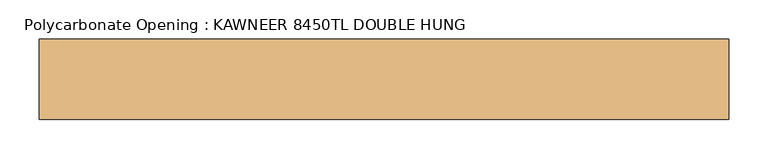
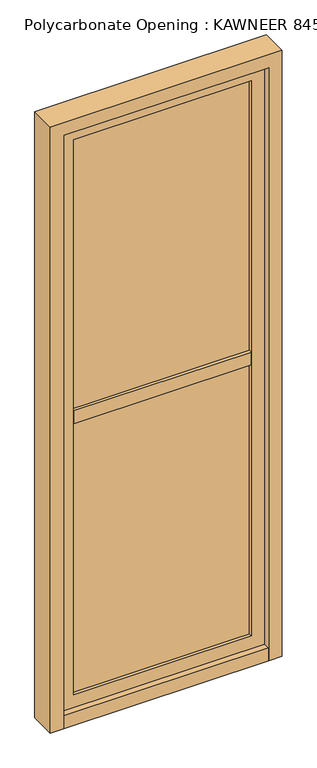
"""IFC4 building model written with IfcOpenShell, lengths in millimetres: door geometry, Polycarbonate Opening : KAWNEER 8450TL DOUBLE HUNG."""

from ifc_helpers import new_model, si_unit, frame, origin, origin_with_axes, place, context, project, spatial, polyline, outline, extrude, source, transform, mapped, element, save


def polycarbonate_opening_kawneer_8450tl_double_hung_174570da(model_context):
    return source(origin(), model_context, "Body", "SweptSolid", [
        extrude(outline(polyline([(386.2916667, -12.7), (-386.2916667, -12.7), (-386.2916667, 12.7), (386.2916667, 12.7), (386.2916667, -12.7)])), frame((0.0, 0.0, 50.8), z_axis=(0.0, 0.0, 1.0), x_axis=(1.0, 0.0, 0.0)), (0.0, 0.0, 1.0), 2311.8580839),
        extrude(outline(polyline([(2362.6580839, -386.2916667), (0.0, -386.2916667), (0.0, 386.2916667), (2362.6580839, 386.2916667), (2362.6580839, -386.2916667)]), holes=[polyline([(101.6, 335.4916667), (101.6, -335.4916667), (2311.8580839, -335.4916667), (2311.8580839, 335.4916667), (101.6, 335.4916667)])]), frame((0.0, -25.4, 0.0), z_axis=(0.0, 1.0, 0.0), x_axis=(0.0, 0.0, 1.0)), (0.0, 0.0, 1.0), 50.8),
        extrude(outline(polyline([(2413.4580839, 437.0916667), (2413.4580839, -437.0916667), (0.0, -437.0916667), (0.0, -386.2916667), (2362.6580839, -386.2916667), (2362.6580839, 386.2916667), (0.0, 386.2916667), (0.0, 437.0916667), (2413.4580839, 437.0916667)])), frame((0.0, -50.8, 0.0), z_axis=(0.0, 1.0, 0.0), x_axis=(0.0, 0.0, 1.0)), (0.0, 0.0, 1.0), 101.6),
        extrude(outline(polyline([(386.2916667, -50.8), (-386.2916667, -50.8), (-386.2916667, 50.8), (386.2916667, 50.8), (386.2916667, -50.8)])), origin_with_axes(), (0.0, 0.0, 1.0), 50.8),
        extrude(outline(polyline([(335.4916667, -25.4), (-335.4916667, -25.4), (-335.4916667, 25.4), (335.4916667, 25.4), (335.4916667, -25.4)])), frame((0.0, 0.0, 1181.329042), z_axis=(0.0, 0.0, 1.0), x_axis=(1.0, 0.0, 0.0)), (0.0, 0.0, 1.0), 50.8),
    ])


if __name__ == "__main__":
    model = new_model("IFC4")
    model_context = context("Model", 3, world=origin())
    ifc_project = project(units=[si_unit("LENGTHUNIT", "METRE", prefix="MILLI")], contexts=[model_context])
    site = spatial("IfcSite", under=ifc_project)
    building = spatial("IfcBuilding", under=site)
    placement = place(None, origin())
    polycarbonate_opening_kawneer_8450tl_double_hung_shape = polycarbonate_opening_kawneer_8450tl_double_hung_174570da(model_context)
    element("IfcDoor", 1, ObjectType="Polycarbonate Opening : KAWNEER 8450TL DOUBLE HUNG", at=placement, inside=building, context=model_context, shape_type="MappedRepresentation", body=[
        mapped(polycarbonate_opening_kawneer_8450tl_double_hung_shape, transform((0.0, 0.0, 0.0), x_axis=(1.0, 0.0, 0.0), y_axis=(0.0, 1.0, 0.0), z_axis=(0.0, 0.0, 1.0))),
    ])
    save(model, "model.ifc")

# Revit data of these elements
# Type "Polycarbonate Opening : KAWNEER 8450TL DOUBLE HUNG"
#   Type Mark = "59"
#   OD_DS_Door_Material = "ALUM./GLAZING"
#   OD_DS_Door_Type = "STOREFRONT - DOUBLE HUNG WINDOW"
#   OD_DS_Lockset = "POLE OPERATOR HARDWARE FOR TOP SASH; BOTTOM SASH MECHANICALLY FIXED"
#   Analytic Construction = "<None>"
#   offset [instance default] = 0' - 2"
#   Stile = 0' - 2"
#   Mullion Width = 0' - 2"
#   Mullion Depth = 0' - 4"
#   Opening Size [instance default] = 5' - 1.50212"
#   Door Width [instance default] = 5' - 1.50212"
#   Window ON/OFF = no
#   Door On/Off = yes
#   Mullion Material = DOUBLE HUNG (CLEAR ANODIZED ALUM) - TEMPERED INSULATED GLAZING (CARDINAL GLASS LoĒ²-240\nOR EQUIVALENT)
#   Glass Material = TEMPERED INSULATED GLAZING (CARDINAL GLASS LoĒ²-240\nOR EQUIVALENT)
#   Door Material = DOUBLE HUNG (CLEAR ANODIZED ALUM) - TEMPERED INSULATED GLAZING (CARDINAL GLASS LoĒ²-240\nOR EQUIVALENT)
# Element 1 (IfcDoor, "Polycarbonate Opening : KAWNEER 8450TL DOUBLE HUNG")
#   offset = 0' - 0"
#   Materials on its faces: "DOUBLE HUNG (CLEAR ANODIZED ALUM) - TEMPERED INSULATED GLAZING (CARDINAL GLASS LoĒ²-240\nOR EQUIVALENT)", "TEMPERED INSULATED GLAZING (CARDINAL GLASS LoĒ²-240\nOR EQUIVALENT)"
# Materials
#   "DOUBLE HUNG (CLEAR ANODIZED ALUM) - TEMPERED INSULATED GLAZING (CARDINAL GLASS LoĒ²-240\nOR EQUIVALENT)": class "Metal", colour RGB 244 244 244, transparency 0, Description = "Aluminum 6061", Cost = 0
#   "TEMPERED INSULATED GLAZING (CARDINAL GLASS LoĒ²-240\nOR EQUIVALENT)": class "Glass", colour RGB 196 205 210, transparency 0.85, Description = "Soda Lime Glass", Cost = 0
